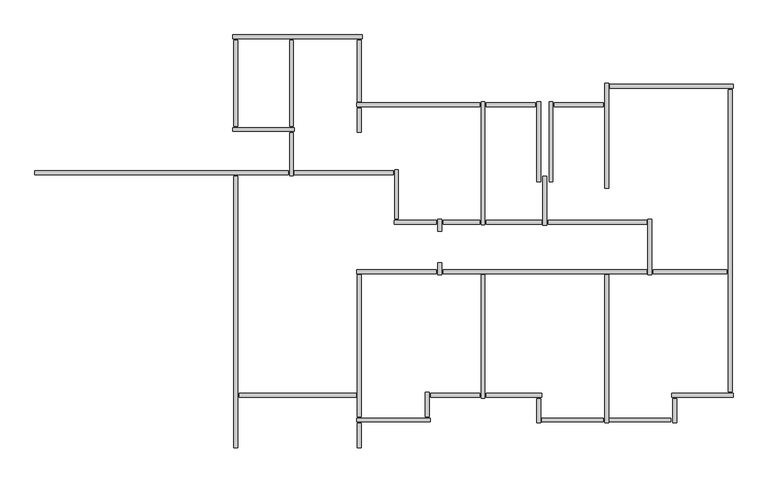
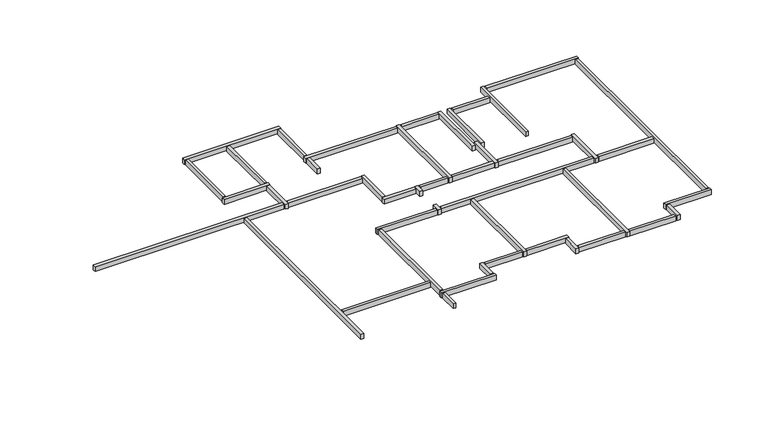
"""IFC4 building model written with IfcOpenShell, lengths in millimetres: beam geometry, Graute viga de respaldo16 : Graute viga de respaldo."""

import ifcopenshell
import ifcopenshell.guid

model = None  # the IFC model being written
_history = None  # IfcOwnerHistory: only IFC2X3 demands one
_inside = {}  # id of a spatial element -> (the spatial element, [elements in it])
_under = {}  # id of a project, library or spatial element -> (it, [spatial elements below it])
_declared = {}  # id of a project -> (the project, [libraries it declares])
_typed = {}  # id of a type object -> (the type object, [elements of that type])
_made_of = {}  # id of a material, layer set ... -> (it, [elements and type objects made of it])


def new_model(schema):
    """Start an empty IFC model of exactly this schema.

    Asked for "IFC4X3", IfcOpenShell would pick the latest addendum, in which some entities
    have other attributes; the version numbers below select the first issue.
    IFC2X3 requires an IfcOwnerHistory on every rooted entity: one is made here for all.
    """
    global model, _history
    if schema == "IFC4X3":
        model = ifcopenshell.file(schema_version=(4, 3, 0, 0))
    else:
        model = ifcopenshell.file(schema=schema)
    _inside.clear()
    _under.clear()
    _declared.clear()
    _typed.clear()
    _made_of.clear()
    _history = None
    if model.schema == "IFC2X3":
        org = make("IfcOrganization", Name="unknown")
        user = make(
            "IfcPersonAndOrganization",
            ThePerson=make("IfcPerson", FamilyName="unknown"),
            TheOrganization=org,
        )
        app = make(
            "IfcApplication",
            ApplicationDeveloper=org,
            Version="unknown",
            ApplicationFullName="unknown",
            ApplicationIdentifier="unknown",
        )
        _history = make(
            "IfcOwnerHistory",
            OwningUser=user,
            OwningApplication=app,
            ChangeAction="ADDED",
            CreationDate=0,
        )
    return model


def make(cls, **values):
    """One entity of the class cls with the attributes given. An attribute that is None is left unset."""
    return model.create_entity(
        cls, **{name: value for name, value in values.items() if value is not None}
    )


def rooted(cls, **values):
    """An entity with a GlobalId (a new one), such as an element, a storey or a relation."""
    return make(cls, GlobalId=ifcopenshell.guid.new(), OwnerHistory=_history, **values)


def si_unit(unit_type, name, prefix=None):
    """IfcSIUnit, for example si_unit("LENGTHUNIT", "METRE", prefix="MILLI")."""
    return make("IfcSIUnit", UnitType=unit_type, Prefix=prefix, Name=name)


def assignment(units):
    """IfcUnitAssignment: the units of a project."""
    return None if units is None else make("IfcUnitAssignment", Units=units)


def point(xyz):
    """IfcCartesianPoint."""
    return None if xyz is None else make("IfcCartesianPoint", Coordinates=xyz)


def direction(xyz):
    """IfcDirection."""
    return None if xyz is None else make("IfcDirection", DirectionRatios=xyz)


def frame(location, z_axis=None, x_axis=None):
    """IfcAxis2Placement3D, a coordinate frame: its origin and axes. An axis left out is left unset."""
    return make(
        "IfcAxis2Placement3D",
        Location=point(location),
        Axis=direction(z_axis),
        RefDirection=direction(x_axis),
    )


def origin():
    """The frame at (0, 0, 0) with its axes left unset."""
    return frame((0.0, 0.0, 0.0))


def place(relative_to, where):
    """IfcLocalPlacement: puts the frame where relative to a parent placement (None: the world)."""
    return make(
        "IfcLocalPlacement", PlacementRelTo=relative_to, RelativePlacement=where
    )


def context(
    kind, dimensions, precision=None, world=None, true_north=None, identifier=None
):
    """IfcGeometricRepresentationContext, for example the 3D "Model" context."""
    return make(
        "IfcGeometricRepresentationContext",
        ContextIdentifier=identifier,
        ContextType=kind,
        CoordinateSpaceDimension=dimensions,
        Precision=precision,
        WorldCoordinateSystem=world,
        TrueNorth=true_north,
    )


def project(units=None, contexts=None):
    """IfcProject with its units and contexts."""
    return rooted(
        "IfcProject",
        Name="project",
        RepresentationContexts=contexts,
        UnitsInContext=assignment(units),
    )


def spatial(cls, under=None, at=None, **own):
    """A site, building, storey or space (cls), placed at a placement, below another one or the project."""
    s = rooted(cls, ObjectPlacement=at, **own)
    if under is not None:
        _under.setdefault(under.id(), (under, []))[1].append(s)
    return s


def polyline(points):
    """IfcPolyline through the points."""
    return make("IfcPolyline", Points=[point(p) for p in points])


def outline(outer, holes=None, kind="AREA"):
    """IfcArbitraryClosedProfileDef: a profile drawn as a closed curve; with holes, ...WithVoids."""
    if holes is None:
        return make("IfcArbitraryClosedProfileDef", ProfileType=kind, OuterCurve=outer)
    return make(
        "IfcArbitraryProfileDefWithVoids",
        ProfileType=kind,
        OuterCurve=outer,
        InnerCurves=holes,
    )


def extrude(swept, where, along, depth):
    """IfcExtrudedAreaSolid: the profile swept, set in the frame where, extruded along a direction by depth."""
    return make(
        "IfcExtrudedAreaSolid",
        SweptArea=swept,
        Position=where,
        ExtrudedDirection=direction(along),
        Depth=depth,
    )


def shape(context_of_items, identifier, shape_type, items):
    """IfcShapeRepresentation: the items that make up one representation, for example the "Body"."""
    return make(
        "IfcShapeRepresentation",
        ContextOfItems=context_of_items,
        RepresentationIdentifier=identifier,
        RepresentationType=shape_type,
        Items=items,
    )


def source(mapping_origin, context_of_items, identifier, shape_type, items):
    """IfcRepresentationMap: a shape defined once, which mapped items show again and again."""
    return make(
        "IfcRepresentationMap",
        MappingOrigin=mapping_origin,
        MappedRepresentation=shape(context_of_items, identifier, shape_type, items),
    )


def transform(
    local_origin,
    x_axis=None,
    y_axis=None,
    z_axis=None,
    scale=None,
    scale2=None,
    scale3=None,
    uniform=True,
):
    """IfcCartesianTransformationOperator3D, or its non-uniform kind. x_axis, y_axis, z_axis: its Axis1, 2, 3."""
    if uniform:
        return make(
            "IfcCartesianTransformationOperator3D",
            Axis1=direction(x_axis),
            Axis2=direction(y_axis),
            LocalOrigin=point(local_origin),
            Scale=scale,
            Axis3=direction(z_axis),
        )
    return make(
        "IfcCartesianTransformationOperator3DnonUniform",
        Axis1=direction(x_axis),
        Axis2=direction(y_axis),
        LocalOrigin=point(local_origin),
        Scale=scale,
        Axis3=direction(z_axis),
        Scale2=scale2,
        Scale3=scale3,
    )


def mapped(mapping_source, mapping_target):
    """IfcMappedItem: shows the shape of a source again, moved by a transform."""
    return make(
        "IfcMappedItem", MappingSource=mapping_source, MappingTarget=mapping_target
    )


def made_of(thing, what):
    """Note that an element or type object is made of a material, layer set ...; save() writes the relation."""
    if what is not None:
        _made_of.setdefault(what.id(), (what, []))[1].append(thing)
    return thing


def element(
    cls,
    number,
    at=None,
    inside=None,
    cuts=None,
    type_object=None,
    material=None,
    context=None,
    identifier="Body",
    shape_type=None,
    held_by="IfcProductDefinitionShape",
    body=None,
    shapes=None,
    **own,
):
    """One element of the class cls, such as IfcWall. Its Tag is "e" and its number.

    at: its placement. inside: the storey or other place that contains it. cuts: it is an
    opening in that element (IfcRelVoidsElement). A single representation is given by context,
    identifier, shape_type and body (its items); several are given by shapes. held_by: the class
    of the entity that holds the representations. save() writes the other relations.
    """
    e = rooted(cls, Tag="e%d" % number, ObjectPlacement=at, **own)
    if body is not None:
        shapes = [shape(context, identifier, shape_type, body)]
    if shapes is not None:
        e.Representation = make(held_by, Representations=shapes)
    if inside is not None:
        _inside.setdefault(inside.id(), (inside, []))[1].append(e)
    if cuts is not None:
        rooted(
            "IfcRelVoidsElement", RelatingBuildingElement=cuts, RelatedOpeningElement=e
        )
    if type_object is not None:
        _typed.setdefault(type_object.id(), (type_object, []))[1].append(e)
    return made_of(e, material)


def aggregate(whole, parts):
    """IfcRelAggregates: a whole, such as a stair, and the parts it consists of."""
    return rooted("IfcRelAggregates", RelatingObject=whole, RelatedObjects=parts)


def save(model, path):
    """Write the relations noted so far, then the file.

    IfcRelAggregates (storeys below a building ...), IfcRelContainedInSpatialStructure (elements
    in a storey), IfcRelDefinesByType, IfcRelAssociatesMaterial and IfcRelDeclares: one each for
    every whole, place, type object, material and project.
    """
    for whole, parts in _under.values():
        aggregate(whole, parts)
    for where, things in _inside.values():
        rooted(
            "IfcRelContainedInSpatialStructure",
            RelatedElements=things,
            RelatingStructure=where,
        )
    for kind, things in _typed.values():
        rooted("IfcRelDefinesByType", RelatedObjects=things, RelatingType=kind)
    for what, things in _made_of.values():
        rooted("IfcRelAssociatesMaterial", RelatedObjects=things, RelatingMaterial=what)
    for by, libraries in _declared.values():
        rooted("IfcRelDeclares", RelatingContext=by, RelatedDefinitions=libraries)
    model.write(path)


def beam_c843057f(model_context):
    return source(origin(), model_context, "Body", "SweptSolid", [
        extrude(outline(polyline([(-54994.9587292, 57408.4278788), (-54994.9587292, 57502.4278788), (-53804.9587292, 57502.4278788), (-53804.9587292, 57408.4278788), (-54994.9587292, 57408.4278788)])), frame((0.0, 0.0, 14632.9999999), z_axis=(0.0, 0.0, 1.0), x_axis=(1.0, 0.0, 0.0)), (0.0, 0.0, 1.0), 167.0),
        extrude(outline(polyline([(-56644.9587292, 57408.4278788), (-56644.9587292, 57502.4278788), (-55454.9587292, 57502.4278788), (-55454.9587292, 57408.4278788), (-56644.9587292, 57408.4278788)])), frame((0.0, 0.0, 14632.9999999), z_axis=(0.0, 0.0, 1.0), x_axis=(1.0, 0.0, 0.0)), (0.0, 0.0, 1.0), 167.0),
        extrude(outline(polyline([(-52594.9587292, 53358.4278788), (-52594.9587292, 53452.4278788), (-50804.9587292, 53452.4278788), (-50804.9587292, 53358.4278788), (-52594.9587292, 53358.4278788)])), frame((0.0, 0.0, 14632.9999999), z_axis=(0.0, 0.0, 1.0), x_axis=(1.0, 0.0, 0.0)), (0.0, 0.0, 1.0), 167.0),
        extrude(outline(polyline([(-57994.9587292, 50358.4278788), (-57994.9587292, 50452.4278788), (-56804.9587292, 50452.4278788), (-56804.9587292, 50358.4278788), (-57994.9587292, 50358.4278788)])), frame((0.0, 0.0, 14632.9999999), z_axis=(0.0, 0.0, 1.0), x_axis=(1.0, 0.0, 0.0)), (0.0, 0.0, 1.0), 167.0),
        extrude(outline(polyline([(-58121.9587292, 50475.4278788), (-58027.9587292, 50475.4278788), (-58027.9587292, 49885.4278788), (-58121.9587292, 49885.4278788), (-58121.9587292, 50475.4278788)])), frame((0.0, 0.0, 14632.9999999), z_axis=(0.0, 0.0, 1.0), x_axis=(1.0, 0.0, 0.0)), (0.0, 0.0, 1.0), 167.0),
        extrude(outline(polyline([(-59794.9587292, 49758.4278788), (-59794.9587292, 49852.4278788), (-58004.9587292, 49852.4278788), (-58004.9587292, 49758.4278788), (-59794.9587292, 49758.4278788)])), frame((0.0, 0.0, 14632.9999999), z_axis=(0.0, 0.0, 1.0), x_axis=(1.0, 0.0, 0.0)), (0.0, 0.0, 1.0), 167.0),
        extrude(outline(polyline([(-57727.9587292, 53335.4278788), (-57821.9587292, 53335.4278788), (-57821.9587292, 53625.4278788), (-57727.9587292, 53625.4278788), (-57727.9587292, 53335.4278788)])), frame((0.0, 0.0, 14632.9999999), z_axis=(0.0, 0.0, 1.0), x_axis=(1.0, 0.0, 0.0)), (0.0, 0.0, 1.0), 167.0),
        extrude(outline(polyline([(-55144.9587292, 54558.4278788), (-55144.9587292, 54652.4278788), (-52754.9587292, 54652.4278788), (-52754.9587292, 54558.4278788), (-55144.9587292, 54558.4278788)])), frame((0.0, 0.0, 14632.9999999), z_axis=(0.0, 0.0, 1.0), x_axis=(1.0, 0.0, 0.0)), (0.0, 0.0, 1.0), 167.0),
        extrude(outline(polyline([(-56644.9587292, 54558.4278788), (-56644.9587292, 54652.4278788), (-55304.9587292, 54652.4278788), (-55304.9587292, 54558.4278788), (-56644.9587292, 54558.4278788)])), frame((0.0, 0.0, 14632.9999999), z_axis=(0.0, 0.0, 1.0), x_axis=(1.0, 0.0, 0.0)), (0.0, 0.0, 1.0), 167.0),
        extrude(outline(polyline([(-57694.9587292, 54558.4278788), (-57694.9587292, 54652.4278788), (-56804.9587292, 54652.4278788), (-56804.9587292, 54558.4278788), (-57694.9587292, 54558.4278788)])), frame((0.0, 0.0, 14632.9999999), z_axis=(0.0, 0.0, 1.0), x_axis=(1.0, 0.0, 0.0)), (0.0, 0.0, 1.0), 167.0),
        extrude(outline(polyline([(-57727.9587292, 54385.4278788), (-57821.9587292, 54385.4278788), (-57821.9587292, 54675.4278788), (-57727.9587292, 54675.4278788), (-57727.9587292, 54385.4278788)])), frame((0.0, 0.0, 14632.9999999), z_axis=(0.0, 0.0, 1.0), x_axis=(1.0, 0.0, 0.0)), (0.0, 0.0, 1.0), 167.0),
        extrude(outline(polyline([(-58884.9587292, 54558.4278788), (-58884.9587292, 54652.4278788), (-57854.9587292, 54652.4278788), (-57854.9587292, 54558.4278788), (-58884.9587292, 54558.4278788)])), frame((0.0, 0.0, 14632.9999999), z_axis=(0.0, 0.0, 1.0), x_axis=(1.0, 0.0, 0.0)), (0.0, 0.0, 1.0), 167.0),
        extrude(outline(polyline([(-58871.9587292, 55875.4278788), (-58777.9587292, 55875.4278788), (-58777.9587292, 54685.4278788), (-58871.9587292, 54685.4278788), (-58871.9587292, 55875.4278788)])), frame((0.0, 0.0, 14632.9999999), z_axis=(0.0, 0.0, 1.0), x_axis=(1.0, 0.0, 0.0)), (0.0, 0.0, 1.0), 167.0),
        extrude(outline(polyline([(-61304.9587292, 55758.4278788), (-61304.9587292, 55852.4278788), (-58904.9587292, 55852.4278788), (-58904.9587292, 55758.4278788), (-61304.9587292, 55758.4278788)])), frame((0.0, 0.0, 14632.9999999), z_axis=(0.0, 0.0, 1.0), x_axis=(1.0, 0.0, 0.0)), (0.0, 0.0, 1.0), 167.0),
        extrude(outline(polyline([(-56677.9587292, 54540.4278788), (-56771.9587292, 54540.4278788), (-56771.9587292, 57525.4278788), (-56677.9587292, 57525.4278788), (-56677.9587292, 54540.4278788)])), frame((0.0, 0.0, 14632.9999999), z_axis=(0.0, 0.0, 1.0), x_axis=(1.0, 0.0, 0.0)), (0.0, 0.0, 1.0), 167.0),
        extrude(outline(polyline([(-59794.9587292, 57408.4278788), (-59794.9587292, 57502.4278788), (-56804.9587292, 57502.4278788), (-56804.9587292, 57408.4278788), (-59794.9587292, 57408.4278788)])), frame((0.0, 0.0, 14632.9999999), z_axis=(0.0, 0.0, 1.0), x_axis=(1.0, 0.0, 0.0)), (0.0, 0.0, 1.0), 167.0),
        extrude(outline(polyline([(-59677.9587292, 56785.4278788), (-59771.9587292, 56785.4278788), (-59771.9587292, 57375.4278788), (-59677.9587292, 57375.4278788), (-59677.9587292, 56785.4278788)])), frame((0.0, 0.0, 14632.9999999), z_axis=(0.0, 0.0, 1.0), x_axis=(1.0, 0.0, 0.0)), (0.0, 0.0, 1.0), 167.0),
        extrude(outline(polyline([(-59771.9587292, 59025.4278788), (-59677.9587292, 59025.4278788), (-59677.9587292, 57535.4278788), (-59771.9587292, 57535.4278788), (-59771.9587292, 59025.4278788)])), frame((0.0, 0.0, 14632.9999999), z_axis=(0.0, 0.0, 1.0), x_axis=(1.0, 0.0, 0.0)), (0.0, 0.0, 1.0), 167.0),
        extrude(outline(polyline([(-62771.9587292, 59025.4278788), (-62677.9587292, 59025.4278788), (-62677.9587292, 56935.4278788), (-62771.9587292, 56935.4278788), (-62771.9587292, 59025.4278788)])), frame((0.0, 0.0, 14632.9999999), z_axis=(0.0, 0.0, 1.0), x_axis=(1.0, 0.0, 0.0)), (0.0, 0.0, 1.0), 167.0),
        extrude(outline(polyline([(-61421.9587292, 59025.4278788), (-61327.9587292, 59025.4278788), (-61327.9587292, 56935.4278788), (-61421.9587292, 56935.4278788), (-61421.9587292, 59025.4278788)])), frame((0.0, 0.0, 14632.9999999), z_axis=(0.0, 0.0, 1.0), x_axis=(1.0, 0.0, 0.0)), (0.0, 0.0, 1.0), 167.0),
        extrude(outline(polyline([(-61327.9587292, 55735.4278788), (-61421.9587292, 55735.4278788), (-61421.9587292, 56775.4278788), (-61327.9587292, 56775.4278788), (-61327.9587292, 55735.4278788)])), frame((0.0, 0.0, 14632.9999999), z_axis=(0.0, 0.0, 1.0), x_axis=(1.0, 0.0, 0.0)), (0.0, 0.0, 1.0), 167.0),
        extrude(outline(polyline([(-62644.9587292, 50358.4278788), (-62644.9587292, 50452.4278788), (-59804.9587292, 50452.4278788), (-59804.9587292, 50358.4278788), (-62644.9587292, 50358.4278788)])), frame((0.0, 0.0, 14632.9999999), z_axis=(0.0, 0.0, 1.0), x_axis=(1.0, 0.0, 0.0)), (0.0, 0.0, 1.0), 167.0),
        extrude(outline(polyline([(-59771.9587292, 53325.4278788), (-59677.9587292, 53325.4278788), (-59677.9587292, 49885.4278788), (-59771.9587292, 49885.4278788), (-59771.9587292, 53325.4278788)])), frame((0.0, 0.0, 14632.9999999), z_axis=(0.0, 0.0, 1.0), x_axis=(1.0, 0.0, 0.0)), (0.0, 0.0, 1.0), 167.0),
        extrude(outline(polyline([(-59794.9587292, 53358.4278788), (-59794.9587292, 53452.4278788), (-57854.9587292, 53452.4278788), (-57854.9587292, 53358.4278788), (-59794.9587292, 53358.4278788)])), frame((0.0, 0.0, 14632.9999999), z_axis=(0.0, 0.0, 1.0), x_axis=(1.0, 0.0, 0.0)), (0.0, 0.0, 1.0), 167.0),
        extrude(outline(polyline([(-57694.9587292, 53358.4278788), (-57694.9587292, 53452.4278788), (-52754.9587292, 53452.4278788), (-52754.9587292, 53358.4278788), (-57694.9587292, 53358.4278788)])), frame((0.0, 0.0, 14632.9999999), z_axis=(0.0, 0.0, 1.0), x_axis=(1.0, 0.0, 0.0)), (0.0, 0.0, 1.0), 167.0),
        extrude(outline(polyline([(-56677.9587292, 50335.4278788), (-56771.9587292, 50335.4278788), (-56771.9587292, 53325.4278788), (-56677.9587292, 53325.4278788), (-56677.9587292, 50335.4278788)])), frame((0.0, 0.0, 14632.9999999), z_axis=(0.0, 0.0, 1.0), x_axis=(1.0, 0.0, 0.0)), (0.0, 0.0, 1.0), 167.0),
        extrude(outline(polyline([(-55304.9587292, 50452.4278788), (-55304.9587292, 50358.4278788), (-56644.9587292, 50358.4278788), (-56644.9587292, 50452.4278788), (-55304.9587292, 50452.4278788)])), frame((0.0, 0.0, 14632.9999999), z_axis=(0.0, 0.0, 1.0), x_axis=(1.0, 0.0, 0.0)), (0.0, 0.0, 1.0), 167.0),
        extrude(outline(polyline([(-55327.9587292, 49735.4278788), (-55421.9587292, 49735.4278788), (-55421.9587292, 50325.4278788), (-55327.9587292, 50325.4278788), (-55327.9587292, 49735.4278788)])), frame((0.0, 0.0, 14632.9999999), z_axis=(0.0, 0.0, 1.0), x_axis=(1.0, 0.0, 0.0)), (0.0, 0.0, 1.0), 167.0),
        extrude(outline(polyline([(-55294.9587292, 49758.4278788), (-55294.9587292, 49852.4278788), (-53804.9587292, 49852.4278788), (-53804.9587292, 49758.4278788), (-55294.9587292, 49758.4278788)])), frame((0.0, 0.0, 14632.9999999), z_axis=(0.0, 0.0, 1.0), x_axis=(1.0, 0.0, 0.0)), (0.0, 0.0, 1.0), 167.0),
        extrude(outline(polyline([(-52165.9809043, 49853.4278788), (-52165.9809043, 49758.4278788), (-53654.9587292, 49758.4278788), (-53654.9587292, 49853.4278788), (-52165.9809043, 49853.4278788)])), frame((0.0, 0.0, 14617.1856208), z_axis=(0.0, 0.0, 1.0), x_axis=(1.0, 0.0, 0.0)), (0.0, 0.0, 1.0), 165.0),
        extrude(outline(polyline([(-50771.9587292, 57825.4278788), (-50677.9587292, 57825.4278788), (-50677.9587292, 50485.4278788), (-50771.9587292, 50485.4278788), (-50771.9587292, 57825.4278788)])), frame((0.0, 0.0, 14632.9999999), z_axis=(0.0, 0.0, 1.0), x_axis=(1.0, 0.0, 0.0)), (0.0, 0.0, 1.0), 167.0),
        extrude(outline(polyline([(-52721.9587292, 54675.4278788), (-52627.9587292, 54675.4278788), (-52627.9587292, 53330.0746661), (-52721.9587292, 53330.0746661), (-52721.9587292, 54675.4278788)])), frame((0.0, 0.0, 14632.9999999), z_axis=(0.0, 0.0, 1.0), x_axis=(1.0, 0.0, 0.0)), (0.0, 0.0, 1.0), 167.0),
        extrude(outline(polyline([(-55271.9587292, 55725.4278788), (-55177.9587292, 55725.4278788), (-55177.9587292, 54535.4278788), (-55271.9587292, 54535.4278788), (-55271.9587292, 55725.4278788)])), frame((0.0, 0.0, 14632.9999999), z_axis=(0.0, 0.0, 1.0), x_axis=(1.0, 0.0, 0.0)), (0.0, 0.0, 1.0), 167.0),
        extrude(outline(polyline([(-55121.9587292, 57525.4278788), (-55027.9587292, 57525.4278788), (-55027.9587292, 55585.4278788), (-55121.9587292, 55585.4278788), (-55121.9587292, 57525.4278788)])), frame((0.0, 0.0, 14632.9999999), z_axis=(0.0, 0.0, 1.0), x_axis=(1.0, 0.0, 0.0)), (0.0, 0.0, 1.0), 167.0),
        extrude(outline(polyline([(-55421.9587292, 57525.4278788), (-55327.9587292, 57525.4278788), (-55327.9587292, 55585.4278788), (-55421.9587292, 55585.4278788), (-55421.9587292, 57525.4278788)])), frame((0.0, 0.0, 14632.9999999), z_axis=(0.0, 0.0, 1.0), x_axis=(1.0, 0.0, 0.0)), (0.0, 0.0, 1.0), 167.0),
        extrude(outline(polyline([(-53771.9587292, 57975.4278788), (-53677.9587292, 57975.4278788), (-53677.9587292, 55435.4278788), (-53771.9587292, 55435.4278788), (-53771.9587292, 57975.4278788)])), frame((0.0, 0.0, 14632.9999999), z_axis=(0.0, 0.0, 1.0), x_axis=(1.0, 0.0, 0.0)), (0.0, 0.0, 1.0), 167.0),
        extrude(outline(polyline([(-50654.9587292, 57952.4278788), (-50654.9587292, 57858.4278788), (-53644.9587292, 57858.4278788), (-53644.9587292, 57952.4278788), (-50654.9587292, 57952.4278788)])), frame((0.0, 0.0, 14632.9999999), z_axis=(0.0, 0.0, 1.0), x_axis=(1.0, 0.0, 0.0)), (0.0, 0.0, 1.0), 167.0),
        extrude(outline(polyline([(-52027.9587292, 49735.4278788), (-52121.9587292, 49735.4278788), (-52121.9587292, 50325.4278788), (-52027.9587292, 50325.4278788), (-52027.9587292, 49735.4278788)])), frame((0.0, 0.0, 14632.9999999), z_axis=(0.0, 0.0, 1.0), x_axis=(1.0, 0.0, 0.0)), (0.0, 0.0, 1.0), 167.0),
        extrude(outline(polyline([(-52144.9587292, 50358.4278788), (-52144.9587292, 50452.4278788), (-50654.9587292, 50452.4278788), (-50654.9587292, 50358.4278788), (-52144.9587292, 50358.4278788)])), frame((0.0, 0.0, 14632.9999999), z_axis=(0.0, 0.0, 1.0), x_axis=(1.0, 0.0, 0.0)), (0.0, 0.0, 1.0), 167.0),
        extrude(outline(polyline([(-53677.9587292, 49735.4278788), (-53771.9587292, 49735.4278788), (-53771.9587292, 53325.4278788), (-53677.9587292, 53325.4278788), (-53677.9587292, 49735.4278788)])), frame((0.0, 0.0, 14632.9999999), z_axis=(0.0, 0.0, 1.0), x_axis=(1.0, 0.0, 0.0)), (0.0, 0.0, 1.0), 167.0),
        extrude(outline(polyline([(-59677.9587292, 49135.4278788), (-59771.9587292, 49135.4278788), (-59771.9587292, 49725.4278788), (-59677.9587292, 49725.4278788), (-59677.9587292, 49135.4278788)])), frame((0.0, 0.0, 14632.9999999), z_axis=(0.0, 0.0, 1.0), x_axis=(1.0, 0.0, 0.0)), (0.0, 0.0, 1.0), 167.0),
        extrude(outline(polyline([(-62794.9587292, 56808.4278788), (-62794.9587292, 56902.4278788), (-61304.9587292, 56902.4278788), (-61304.9587292, 56808.4278788), (-62794.9587292, 56808.4278788)])), frame((0.0, 0.0, 14632.9999999), z_axis=(0.0, 0.0, 1.0), x_axis=(1.0, 0.0, 0.0)), (0.0, 0.0, 1.0), 167.0),
        extrude(outline(polyline([(-62794.9587292, 59058.4278788), (-62794.9587292, 59152.4278788), (-59654.9587292, 59152.4278788), (-59654.9587292, 59058.4278788), (-62794.9587292, 59058.4278788)])), frame((0.0, 0.0, 14632.9999999), z_axis=(0.0, 0.0, 1.0), x_axis=(1.0, 0.0, 0.0)), (0.0, 0.0, 1.0), 167.0),
        extrude(outline(polyline([(-67601.7587292, 55758.4278788), (-67601.7587292, 55852.4278788), (-61454.9587292, 55852.4278788), (-61454.9587292, 55758.4278788), (-67601.7587292, 55758.4278788)])), frame((0.0, 0.0, 14632.9999999), z_axis=(0.0, 0.0, 1.0), x_axis=(1.0, 0.0, 0.0)), (0.0, 0.0, 1.0), 167.0),
        extrude(outline(polyline([(-62677.9587292, 49132.8979841), (-62771.9587292, 49132.8979841), (-62771.9587292, 55725.4278788), (-62677.9587292, 55725.4278788), (-62677.9587292, 49132.8979841)])), frame((0.0, 0.0, 14632.9999999), z_axis=(0.0, 0.0, 1.0), x_axis=(1.0, 0.0, 0.0)), (0.0, 0.0, 1.0), 167.0),
    ])


if __name__ == "__main__":
    model = new_model("IFC4")
    model_context = context("Model", 3, world=origin())
    ifc_project = project(units=[si_unit("LENGTHUNIT", "METRE", prefix="MILLI")], contexts=[model_context])
    site = spatial("IfcSite", under=ifc_project)
    building = spatial("IfcBuilding", under=site)
    placement = place(None, origin())
    beam_shape = beam_c843057f(model_context)
    element("IfcBeam", 1, ObjectType="Graute viga de respaldo16 : Graute viga de respaldo", at=placement, inside=building, context=model_context, shape_type="MappedRepresentation", body=[
        mapped(beam_shape, transform((0.0, 0.0, 0.0), x_axis=(1.0, 0.0, 0.0), y_axis=(0.0, 1.0, 0.0), z_axis=(0.0, 0.0, 1.0))),
    ])
    save(model, "model.ifc")

# Revit data of these elements
# Element 1 (IfcBeam, "Graute viga de respaldo16 : Graute viga de respaldo")
#   Materials on its faces: "Concreto, Faixa de areia/cimento"
# Materials
#   "Concreto, Faixa de areia/cimento": class "Concreto", colour RGB 127 127 127, transparency 0, Description = "Revestimento de laje de concreto", Cost = 0
